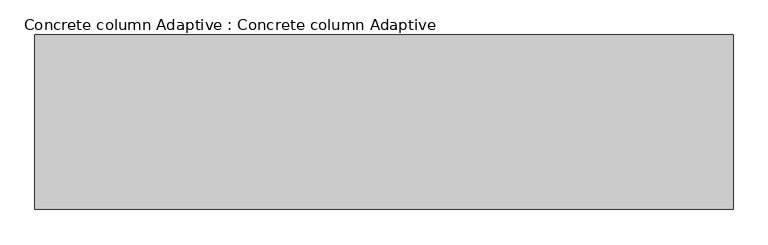
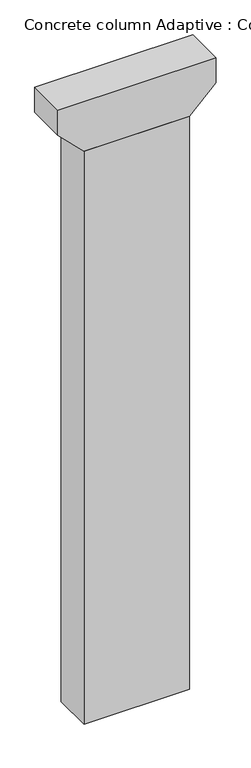
"""IFC4 building model written with IfcOpenShell, lengths in millimetres: proxy geometry, Concrete column Adaptive : Concrete column Adaptive."""

import ifcopenshell
import ifcopenshell.guid

model = None  # the IFC model being written
_history = None  # IfcOwnerHistory: only IFC2X3 demands one
_inside = {}  # id of a spatial element -> (the spatial element, [elements in it])
_under = {}  # id of a project, library or spatial element -> (it, [spatial elements below it])
_declared = {}  # id of a project -> (the project, [libraries it declares])
_typed = {}  # id of a type object -> (the type object, [elements of that type])
_made_of = {}  # id of a material, layer set ... -> (it, [elements and type objects made of it])


def new_model(schema):
    """Start an empty IFC model of exactly this schema.

    Asked for "IFC4X3", IfcOpenShell would pick the latest addendum, in which some entities
    have other attributes; the version numbers below select the first issue.
    IFC2X3 requires an IfcOwnerHistory on every rooted entity: one is made here for all.
    """
    global model, _history
    if schema == "IFC4X3":
        model = ifcopenshell.file(schema_version=(4, 3, 0, 0))
    else:
        model = ifcopenshell.file(schema=schema)
    _inside.clear()
    _under.clear()
    _declared.clear()
    _typed.clear()
    _made_of.clear()
    _history = None
    if model.schema == "IFC2X3":
        org = make("IfcOrganization", Name="unknown")
        user = make(
            "IfcPersonAndOrganization",
            ThePerson=make("IfcPerson", FamilyName="unknown"),
            TheOrganization=org,
        )
        app = make(
            "IfcApplication",
            ApplicationDeveloper=org,
            Version="unknown",
            ApplicationFullName="unknown",
            ApplicationIdentifier="unknown",
        )
        _history = make(
            "IfcOwnerHistory",
            OwningUser=user,
            OwningApplication=app,
            ChangeAction="ADDED",
            CreationDate=0,
        )
    return model


def make(cls, **values):
    """One entity of the class cls with the attributes given. An attribute that is None is left unset."""
    return model.create_entity(
        cls, **{name: value for name, value in values.items() if value is not None}
    )


def rooted(cls, **values):
    """An entity with a GlobalId (a new one), such as an element, a storey or a relation."""
    return make(cls, GlobalId=ifcopenshell.guid.new(), OwnerHistory=_history, **values)


def si_unit(unit_type, name, prefix=None):
    """IfcSIUnit, for example si_unit("LENGTHUNIT", "METRE", prefix="MILLI")."""
    return make("IfcSIUnit", UnitType=unit_type, Prefix=prefix, Name=name)


def assignment(units):
    """IfcUnitAssignment: the units of a project."""
    return None if units is None else make("IfcUnitAssignment", Units=units)


def point(xyz):
    """IfcCartesianPoint."""
    return None if xyz is None else make("IfcCartesianPoint", Coordinates=xyz)


def direction(xyz):
    """IfcDirection."""
    return None if xyz is None else make("IfcDirection", DirectionRatios=xyz)


def frame(location, z_axis=None, x_axis=None):
    """IfcAxis2Placement3D, a coordinate frame: its origin and axes. An axis left out is left unset."""
    return make(
        "IfcAxis2Placement3D",
        Location=point(location),
        Axis=direction(z_axis),
        RefDirection=direction(x_axis),
    )


def origin():
    """The frame at (0, 0, 0) with its axes left unset."""
    return frame((0.0, 0.0, 0.0))


def origin_with_axes():
    """The frame at (0, 0, 0) with the z axis (0, 0, 1) and the x axis (1, 0, 0) written out."""
    return frame((0.0, 0.0, 0.0), z_axis=(0.0, 0.0, 1.0), x_axis=(1.0, 0.0, 0.0))


def place(relative_to, where):
    """IfcLocalPlacement: puts the frame where relative to a parent placement (None: the world)."""
    return make(
        "IfcLocalPlacement", PlacementRelTo=relative_to, RelativePlacement=where
    )


def context(
    kind, dimensions, precision=None, world=None, true_north=None, identifier=None
):
    """IfcGeometricRepresentationContext, for example the 3D "Model" context."""
    return make(
        "IfcGeometricRepresentationContext",
        ContextIdentifier=identifier,
        ContextType=kind,
        CoordinateSpaceDimension=dimensions,
        Precision=precision,
        WorldCoordinateSystem=world,
        TrueNorth=true_north,
    )


def project(units=None, contexts=None):
    """IfcProject with its units and contexts."""
    return rooted(
        "IfcProject",
        Name="project",
        RepresentationContexts=contexts,
        UnitsInContext=assignment(units),
    )


def spatial(cls, under=None, at=None, **own):
    """A site, building, storey or space (cls), placed at a placement, below another one or the project."""
    s = rooted(cls, ObjectPlacement=at, **own)
    if under is not None:
        _under.setdefault(under.id(), (under, []))[1].append(s)
    return s


def polyline(points):
    """IfcPolyline through the points."""
    return make("IfcPolyline", Points=[point(p) for p in points])


def outline(outer, holes=None, kind="AREA"):
    """IfcArbitraryClosedProfileDef: a profile drawn as a closed curve; with holes, ...WithVoids."""
    if holes is None:
        return make("IfcArbitraryClosedProfileDef", ProfileType=kind, OuterCurve=outer)
    return make(
        "IfcArbitraryProfileDefWithVoids",
        ProfileType=kind,
        OuterCurve=outer,
        InnerCurves=holes,
    )


def extrude(swept, where, along, depth):
    """IfcExtrudedAreaSolid: the profile swept, set in the frame where, extruded along a direction by depth."""
    return make(
        "IfcExtrudedAreaSolid",
        SweptArea=swept,
        Position=where,
        ExtrudedDirection=direction(along),
        Depth=depth,
    )


def shape(context_of_items, identifier, shape_type, items):
    """IfcShapeRepresentation: the items that make up one representation, for example the "Body"."""
    return make(
        "IfcShapeRepresentation",
        ContextOfItems=context_of_items,
        RepresentationIdentifier=identifier,
        RepresentationType=shape_type,
        Items=items,
    )


def source(mapping_origin, context_of_items, identifier, shape_type, items):
    """IfcRepresentationMap: a shape defined once, which mapped items show again and again."""
    return make(
        "IfcRepresentationMap",
        MappingOrigin=mapping_origin,
        MappedRepresentation=shape(context_of_items, identifier, shape_type, items),
    )


def transform(
    local_origin,
    x_axis=None,
    y_axis=None,
    z_axis=None,
    scale=None,
    scale2=None,
    scale3=None,
    uniform=True,
):
    """IfcCartesianTransformationOperator3D, or its non-uniform kind. x_axis, y_axis, z_axis: its Axis1, 2, 3."""
    if uniform:
        return make(
            "IfcCartesianTransformationOperator3D",
            Axis1=direction(x_axis),
            Axis2=direction(y_axis),
            LocalOrigin=point(local_origin),
            Scale=scale,
            Axis3=direction(z_axis),
        )
    return make(
        "IfcCartesianTransformationOperator3DnonUniform",
        Axis1=direction(x_axis),
        Axis2=direction(y_axis),
        LocalOrigin=point(local_origin),
        Scale=scale,
        Axis3=direction(z_axis),
        Scale2=scale2,
        Scale3=scale3,
    )


def mapped(mapping_source, mapping_target):
    """IfcMappedItem: shows the shape of a source again, moved by a transform."""
    return make(
        "IfcMappedItem", MappingSource=mapping_source, MappingTarget=mapping_target
    )


def made_of(thing, what):
    """Note that an element or type object is made of a material, layer set ...; save() writes the relation."""
    if what is not None:
        _made_of.setdefault(what.id(), (what, []))[1].append(thing)
    return thing


def element(
    cls,
    number,
    at=None,
    inside=None,
    cuts=None,
    type_object=None,
    material=None,
    context=None,
    identifier="Body",
    shape_type=None,
    held_by="IfcProductDefinitionShape",
    body=None,
    shapes=None,
    **own,
):
    """One element of the class cls, such as IfcWall. Its Tag is "e" and its number.

    at: its placement. inside: the storey or other place that contains it. cuts: it is an
    opening in that element (IfcRelVoidsElement). A single representation is given by context,
    identifier, shape_type and body (its items); several are given by shapes. held_by: the class
    of the entity that holds the representations. save() writes the other relations.
    """
    e = rooted(cls, Tag="e%d" % number, ObjectPlacement=at, **own)
    if body is not None:
        shapes = [shape(context, identifier, shape_type, body)]
    if shapes is not None:
        e.Representation = make(held_by, Representations=shapes)
    if inside is not None:
        _inside.setdefault(inside.id(), (inside, []))[1].append(e)
    if cuts is not None:
        rooted(
            "IfcRelVoidsElement", RelatingBuildingElement=cuts, RelatedOpeningElement=e
        )
    if type_object is not None:
        _typed.setdefault(type_object.id(), (type_object, []))[1].append(e)
    return made_of(e, material)


def aggregate(whole, parts):
    """IfcRelAggregates: a whole, such as a stair, and the parts it consists of."""
    return rooted("IfcRelAggregates", RelatingObject=whole, RelatedObjects=parts)


def save(model, path):
    """Write the relations noted so far, then the file.

    IfcRelAggregates (storeys below a building ...), IfcRelContainedInSpatialStructure (elements
    in a storey), IfcRelDefinesByType, IfcRelAssociatesMaterial and IfcRelDeclares: one each for
    every whole, place, type object, material and project.
    """
    for whole, parts in _under.values():
        aggregate(whole, parts)
    for where, things in _inside.values():
        rooted(
            "IfcRelContainedInSpatialStructure",
            RelatedElements=things,
            RelatingStructure=where,
        )
    for kind, things in _typed.values():
        rooted("IfcRelDefinesByType", RelatedObjects=things, RelatingType=kind)
    for what, things in _made_of.values():
        rooted("IfcRelAssociatesMaterial", RelatedObjects=things, RelatingMaterial=what)
    for by, libraries in _declared.values():
        rooted("IfcRelDeclares", RelatingContext=by, RelatedDefinitions=libraries)
    model.write(path)


def concrete_column_adaptive_concrete_column_adaptive_a8665295(model_context):
    return source(origin(), model_context, "Body", "SweptSolid", [
        extrude(outline(polyline([(49912.0, 6000.0), (49912.0, -6000.0), (47912.0, -6000.0), (45912.0, -4000.0), (45912.0, 4000.0), (47912.0, 6000.0), (49912.0, 6000.0)])), frame((0.0, -1500.0, 0.0), z_axis=(0.0, 1.0, 0.0), x_axis=(0.0, 0.0, 1.0)), (0.0, 0.0, 1.0), 3000.0),
        extrude(outline(polyline([(-4000.0, -1500.0), (-4000.0, 1500.0), (4000.0, 1500.0), (4000.0, -1500.0), (-4000.0, -1500.0)])), origin_with_axes(), (0.0, 0.0, 1.0), 45912.0),
    ])


if __name__ == "__main__":
    model = new_model("IFC4")
    model_context = context("Model", 3, world=origin())
    ifc_project = project(units=[si_unit("LENGTHUNIT", "METRE", prefix="MILLI")], contexts=[model_context])
    site = spatial("IfcSite", under=ifc_project)
    building = spatial("IfcBuilding", under=site)
    placement = place(None, origin())
    concrete_column_adaptive_concrete_column_adaptive_shape = concrete_column_adaptive_concrete_column_adaptive_a8665295(model_context)
    element("IfcBuildingElementProxy", 1, Name="Concrete column Adaptive : Concrete column Adaptive", ObjectType="Concrete column Adaptive : Concrete column Adaptive", at=placement, inside=building, context=model_context, shape_type="MappedRepresentation", body=[
        mapped(concrete_column_adaptive_concrete_column_adaptive_shape, transform((0.0, 0.0, 0.0), x_axis=(1.0, 0.0, 0.0), y_axis=(0.0, 1.0, 0.0), z_axis=(0.0, 0.0, 1.0))),
    ])
    save(model, "model.ifc")

# Revit data of these elements
# Type "Concrete column Adaptive : Concrete column Adaptive"
#   Height [instance default] = 30000 mm
#   Default Elevation = 0
# Element 1 (IfcBuildingElementProxy, "Concrete column Adaptive : Concrete column Adaptive")
#   Height = 45912 mm
